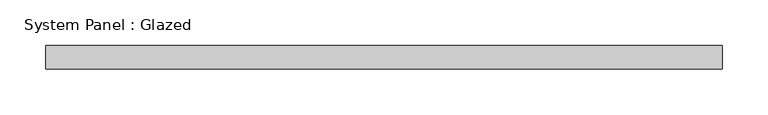
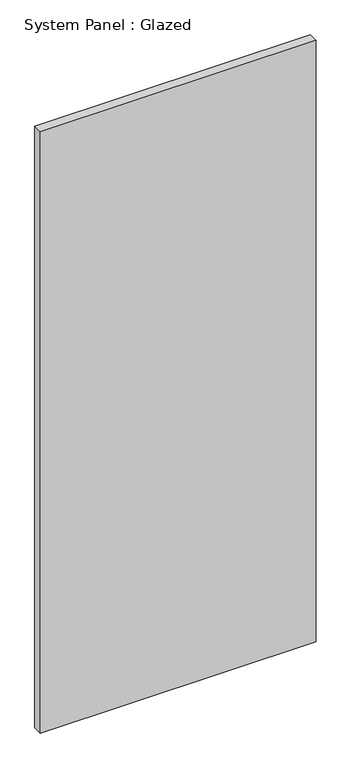
"""IFC4 building model written with IfcOpenShell, lengths in millimetres: plate geometry, System Panel : Glazed."""

from ifc_helpers import new_model, si_unit, origin, origin_with_axes, place, context, project, spatial, polyline, outline, extrude, source, transform, mapped, element, save


def system_panel_glazed_6a423235(model_context):
    return source(origin(), model_context, "Body", "SweptSolid", [
        extrude(outline(polyline([(369.0416667, 19.05), (-369.0416667, 19.05), (-369.0416667, 44.45), (369.0416667, 44.45), (369.0416667, 19.05)])), origin_with_axes(), (0.0, 0.0, 1.0), 1701.8),
    ])


if __name__ == "__main__":
    model = new_model("IFC4")
    model_context = context("Model", 3, world=origin())
    ifc_project = project(units=[si_unit("LENGTHUNIT", "METRE", prefix="MILLI")], contexts=[model_context])
    site = spatial("IfcSite", under=ifc_project)
    building = spatial("IfcBuilding", under=site)
    placement = place(None, origin())
    system_panel_glazed_shape = system_panel_glazed_6a423235(model_context)
    element("IfcPlate", 1, ObjectType="System Panel : Glazed", at=placement, inside=building, context=model_context, shape_type="MappedRepresentation", body=[
        mapped(system_panel_glazed_shape, transform((0.0, 0.0, 0.0), x_axis=(1.0, 0.0, 0.0), y_axis=(0.0, 1.0, 0.0), z_axis=(0.0, 0.0, 1.0))),
    ])
    save(model, "model.ifc")

# Revit data of these elements
# Element 1 (IfcPlate, "System Panel : Glazed")
#   Materials on its faces: "Glass"
# Materials
#   "Glass": class "Glass", colour RGB 0 128 192, transparency 0.75
